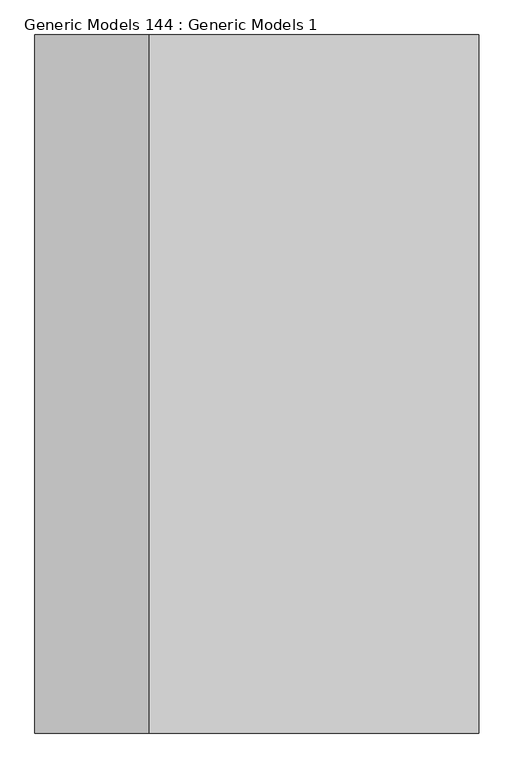
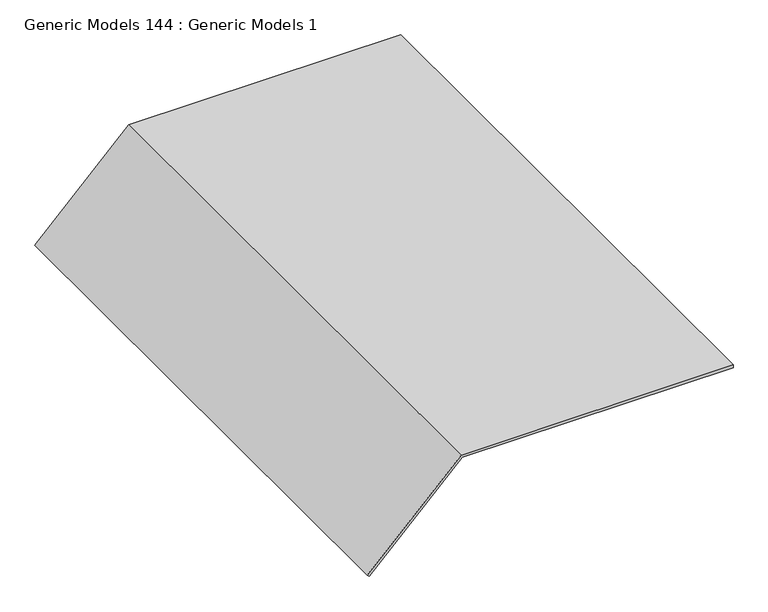
"""IFC4 building model written with IfcOpenShell, lengths in millimetres: proxy geometry, Generic Models 144 : Generic Models 1."""

import ifcopenshell
import ifcopenshell.guid

model = None  # the IFC model being written
_history = None  # IfcOwnerHistory: only IFC2X3 demands one
_inside = {}  # id of a spatial element -> (the spatial element, [elements in it])
_under = {}  # id of a project, library or spatial element -> (it, [spatial elements below it])
_declared = {}  # id of a project -> (the project, [libraries it declares])
_typed = {}  # id of a type object -> (the type object, [elements of that type])
_made_of = {}  # id of a material, layer set ... -> (it, [elements and type objects made of it])


def new_model(schema):
    """Start an empty IFC model of exactly this schema.

    Asked for "IFC4X3", IfcOpenShell would pick the latest addendum, in which some entities
    have other attributes; the version numbers below select the first issue.
    IFC2X3 requires an IfcOwnerHistory on every rooted entity: one is made here for all.
    """
    global model, _history
    if schema == "IFC4X3":
        model = ifcopenshell.file(schema_version=(4, 3, 0, 0))
    else:
        model = ifcopenshell.file(schema=schema)
    _inside.clear()
    _under.clear()
    _declared.clear()
    _typed.clear()
    _made_of.clear()
    _history = None
    if model.schema == "IFC2X3":
        org = make("IfcOrganization", Name="unknown")
        user = make(
            "IfcPersonAndOrganization",
            ThePerson=make("IfcPerson", FamilyName="unknown"),
            TheOrganization=org,
        )
        app = make(
            "IfcApplication",
            ApplicationDeveloper=org,
            Version="unknown",
            ApplicationFullName="unknown",
            ApplicationIdentifier="unknown",
        )
        _history = make(
            "IfcOwnerHistory",
            OwningUser=user,
            OwningApplication=app,
            ChangeAction="ADDED",
            CreationDate=0,
        )
    return model


def make(cls, **values):
    """One entity of the class cls with the attributes given. An attribute that is None is left unset."""
    return model.create_entity(
        cls, **{name: value for name, value in values.items() if value is not None}
    )


def rooted(cls, **values):
    """An entity with a GlobalId (a new one), such as an element, a storey or a relation."""
    return make(cls, GlobalId=ifcopenshell.guid.new(), OwnerHistory=_history, **values)


def si_unit(unit_type, name, prefix=None):
    """IfcSIUnit, for example si_unit("LENGTHUNIT", "METRE", prefix="MILLI")."""
    return make("IfcSIUnit", UnitType=unit_type, Prefix=prefix, Name=name)


def assignment(units):
    """IfcUnitAssignment: the units of a project."""
    return None if units is None else make("IfcUnitAssignment", Units=units)


def point(xyz):
    """IfcCartesianPoint."""
    return None if xyz is None else make("IfcCartesianPoint", Coordinates=xyz)


def direction(xyz):
    """IfcDirection."""
    return None if xyz is None else make("IfcDirection", DirectionRatios=xyz)


def frame(location, z_axis=None, x_axis=None):
    """IfcAxis2Placement3D, a coordinate frame: its origin and axes. An axis left out is left unset."""
    return make(
        "IfcAxis2Placement3D",
        Location=point(location),
        Axis=direction(z_axis),
        RefDirection=direction(x_axis),
    )


def origin():
    """The frame at (0, 0, 0) with its axes left unset."""
    return frame((0.0, 0.0, 0.0))


def place(relative_to, where):
    """IfcLocalPlacement: puts the frame where relative to a parent placement (None: the world)."""
    return make(
        "IfcLocalPlacement", PlacementRelTo=relative_to, RelativePlacement=where
    )


def context(
    kind, dimensions, precision=None, world=None, true_north=None, identifier=None
):
    """IfcGeometricRepresentationContext, for example the 3D "Model" context."""
    return make(
        "IfcGeometricRepresentationContext",
        ContextIdentifier=identifier,
        ContextType=kind,
        CoordinateSpaceDimension=dimensions,
        Precision=precision,
        WorldCoordinateSystem=world,
        TrueNorth=true_north,
    )


def project(units=None, contexts=None):
    """IfcProject with its units and contexts."""
    return rooted(
        "IfcProject",
        Name="project",
        RepresentationContexts=contexts,
        UnitsInContext=assignment(units),
    )


def spatial(cls, under=None, at=None, **own):
    """A site, building, storey or space (cls), placed at a placement, below another one or the project."""
    s = rooted(cls, ObjectPlacement=at, **own)
    if under is not None:
        _under.setdefault(under.id(), (under, []))[1].append(s)
    return s


def polyline(points):
    """IfcPolyline through the points."""
    return make("IfcPolyline", Points=[point(p) for p in points])


def outline(outer, holes=None, kind="AREA"):
    """IfcArbitraryClosedProfileDef: a profile drawn as a closed curve; with holes, ...WithVoids."""
    if holes is None:
        return make("IfcArbitraryClosedProfileDef", ProfileType=kind, OuterCurve=outer)
    return make(
        "IfcArbitraryProfileDefWithVoids",
        ProfileType=kind,
        OuterCurve=outer,
        InnerCurves=holes,
    )


def extrude(swept, where, along, depth):
    """IfcExtrudedAreaSolid: the profile swept, set in the frame where, extruded along a direction by depth."""
    return make(
        "IfcExtrudedAreaSolid",
        SweptArea=swept,
        Position=where,
        ExtrudedDirection=direction(along),
        Depth=depth,
    )


def shape(context_of_items, identifier, shape_type, items):
    """IfcShapeRepresentation: the items that make up one representation, for example the "Body"."""
    return make(
        "IfcShapeRepresentation",
        ContextOfItems=context_of_items,
        RepresentationIdentifier=identifier,
        RepresentationType=shape_type,
        Items=items,
    )


def source(mapping_origin, context_of_items, identifier, shape_type, items):
    """IfcRepresentationMap: a shape defined once, which mapped items show again and again."""
    return make(
        "IfcRepresentationMap",
        MappingOrigin=mapping_origin,
        MappedRepresentation=shape(context_of_items, identifier, shape_type, items),
    )


def transform(
    local_origin,
    x_axis=None,
    y_axis=None,
    z_axis=None,
    scale=None,
    scale2=None,
    scale3=None,
    uniform=True,
):
    """IfcCartesianTransformationOperator3D, or its non-uniform kind. x_axis, y_axis, z_axis: its Axis1, 2, 3."""
    if uniform:
        return make(
            "IfcCartesianTransformationOperator3D",
            Axis1=direction(x_axis),
            Axis2=direction(y_axis),
            LocalOrigin=point(local_origin),
            Scale=scale,
            Axis3=direction(z_axis),
        )
    return make(
        "IfcCartesianTransformationOperator3DnonUniform",
        Axis1=direction(x_axis),
        Axis2=direction(y_axis),
        LocalOrigin=point(local_origin),
        Scale=scale,
        Axis3=direction(z_axis),
        Scale2=scale2,
        Scale3=scale3,
    )


def mapped(mapping_source, mapping_target):
    """IfcMappedItem: shows the shape of a source again, moved by a transform."""
    return make(
        "IfcMappedItem", MappingSource=mapping_source, MappingTarget=mapping_target
    )


def made_of(thing, what):
    """Note that an element or type object is made of a material, layer set ...; save() writes the relation."""
    if what is not None:
        _made_of.setdefault(what.id(), (what, []))[1].append(thing)
    return thing


def element(
    cls,
    number,
    at=None,
    inside=None,
    cuts=None,
    type_object=None,
    material=None,
    context=None,
    identifier="Body",
    shape_type=None,
    held_by="IfcProductDefinitionShape",
    body=None,
    shapes=None,
    **own,
):
    """One element of the class cls, such as IfcWall. Its Tag is "e" and its number.

    at: its placement. inside: the storey or other place that contains it. cuts: it is an
    opening in that element (IfcRelVoidsElement). A single representation is given by context,
    identifier, shape_type and body (its items); several are given by shapes. held_by: the class
    of the entity that holds the representations. save() writes the other relations.
    """
    e = rooted(cls, Tag="e%d" % number, ObjectPlacement=at, **own)
    if body is not None:
        shapes = [shape(context, identifier, shape_type, body)]
    if shapes is not None:
        e.Representation = make(held_by, Representations=shapes)
    if inside is not None:
        _inside.setdefault(inside.id(), (inside, []))[1].append(e)
    if cuts is not None:
        rooted(
            "IfcRelVoidsElement", RelatingBuildingElement=cuts, RelatedOpeningElement=e
        )
    if type_object is not None:
        _typed.setdefault(type_object.id(), (type_object, []))[1].append(e)
    return made_of(e, material)


def aggregate(whole, parts):
    """IfcRelAggregates: a whole, such as a stair, and the parts it consists of."""
    return rooted("IfcRelAggregates", RelatingObject=whole, RelatedObjects=parts)


def save(model, path):
    """Write the relations noted so far, then the file.

    IfcRelAggregates (storeys below a building ...), IfcRelContainedInSpatialStructure (elements
    in a storey), IfcRelDefinesByType, IfcRelAssociatesMaterial and IfcRelDeclares: one each for
    every whole, place, type object, material and project.
    """
    for whole, parts in _under.values():
        aggregate(whole, parts)
    for where, things in _inside.values():
        rooted(
            "IfcRelContainedInSpatialStructure",
            RelatedElements=things,
            RelatingStructure=where,
        )
    for kind, things in _typed.values():
        rooted("IfcRelDefinesByType", RelatedObjects=things, RelatingType=kind)
    for what, things in _made_of.values():
        rooted("IfcRelAssociatesMaterial", RelatedObjects=things, RelatingMaterial=what)
    for by, libraries in _declared.values():
        rooted("IfcRelDeclares", RelatingContext=by, RelatedDefinitions=libraries)
    model.write(path)


def generic_models_144_generic_models_1_4ebe4832(model_context):
    return source(origin(), model_context, "Body", "SweptSolid", [
        extrude(outline(polyline([(-79.375, 52785.9625), (-73.025, 52785.9625), (-73.025, 52209.6280698), (-272.1843039, 52010.4687659), (-276.674432, 52014.9588939), (-79.375, 52212.2583259), (-79.375, 52785.9625)])), frame((0.0, 0.0, 0.0), z_axis=(0.0, 1.0, 0.0), x_axis=(0.0, 0.0, 1.0)), (0.0, 0.0, 1.0), 1219.2),
    ])


if __name__ == "__main__":
    model = new_model("IFC4")
    model_context = context("Model", 3, world=origin())
    ifc_project = project(units=[si_unit("LENGTHUNIT", "METRE", prefix="MILLI")], contexts=[model_context])
    site = spatial("IfcSite", under=ifc_project)
    building = spatial("IfcBuilding", under=site)
    placement = place(None, origin())
    generic_models_144_generic_models_1_shape = generic_models_144_generic_models_1_4ebe4832(model_context)
    element("IfcBuildingElementProxy", 1, Name="Generic Models 144 : Generic Models 1", ObjectType="Generic Models 144 : Generic Models 1", at=placement, inside=building, context=model_context, shape_type="MappedRepresentation", body=[
        mapped(generic_models_144_generic_models_1_shape, transform((0.0, 0.0, 0.0), x_axis=(1.0, 0.0, 0.0), y_axis=(0.0, 1.0, 0.0), z_axis=(0.0, 0.0, 1.0))),
    ])
    save(model, "model.ifc")

# Revit data of these elements
# Element 1 (IfcBuildingElementProxy, "Generic Models 144 : Generic Models 1")
#   Materials on its faces: "#10 6x6 WIRE MESH"
# Materials
#   "#10 6x6 WIRE MESH": class "Metal", colour RGB 189 187 185, transparency 0, Description = "Structural steel 50ksi", Cost = 0
